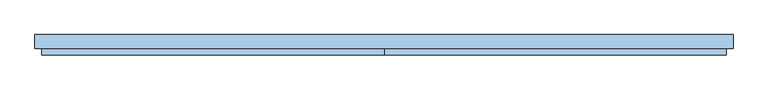
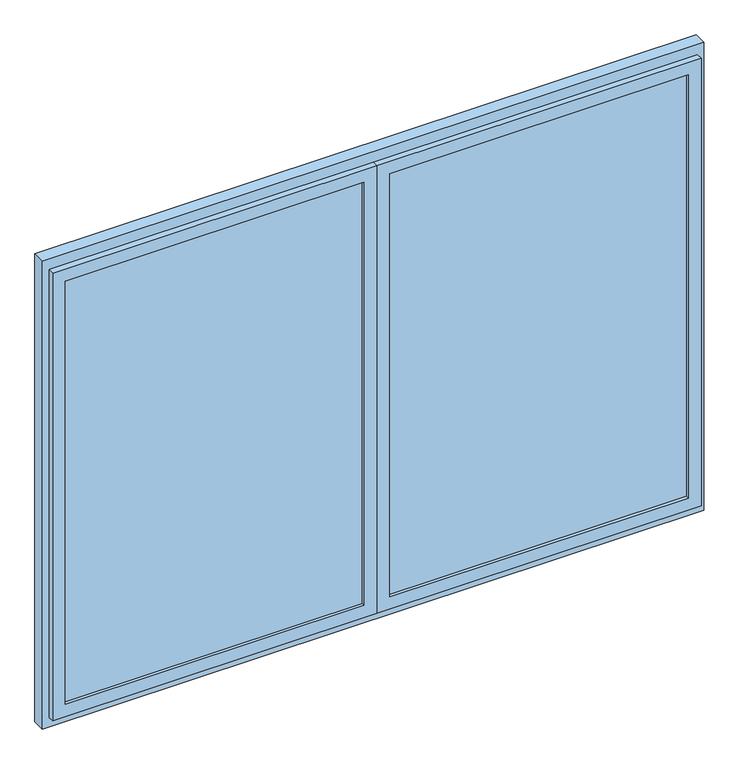
"""IFC4 building model written with IfcOpenShell, lengths in millimetres: window geometry, Fenstertür 2-flg : Fenstertür 2-flg 3.075x2.3."""

import ifcopenshell
import ifcopenshell.guid

model = None  # the IFC model being written
_history = None  # IfcOwnerHistory: only IFC2X3 demands one
_inside = {}  # id of a spatial element -> (the spatial element, [elements in it])
_under = {}  # id of a project, library or spatial element -> (it, [spatial elements below it])
_declared = {}  # id of a project -> (the project, [libraries it declares])
_typed = {}  # id of a type object -> (the type object, [elements of that type])
_made_of = {}  # id of a material, layer set ... -> (it, [elements and type objects made of it])


def new_model(schema):
    """Start an empty IFC model of exactly this schema.

    Asked for "IFC4X3", IfcOpenShell would pick the latest addendum, in which some entities
    have other attributes; the version numbers below select the first issue.
    IFC2X3 requires an IfcOwnerHistory on every rooted entity: one is made here for all.
    """
    global model, _history
    if schema == "IFC4X3":
        model = ifcopenshell.file(schema_version=(4, 3, 0, 0))
    else:
        model = ifcopenshell.file(schema=schema)
    _inside.clear()
    _under.clear()
    _declared.clear()
    _typed.clear()
    _made_of.clear()
    _history = None
    if model.schema == "IFC2X3":
        org = make("IfcOrganization", Name="unknown")
        user = make(
            "IfcPersonAndOrganization",
            ThePerson=make("IfcPerson", FamilyName="unknown"),
            TheOrganization=org,
        )
        app = make(
            "IfcApplication",
            ApplicationDeveloper=org,
            Version="unknown",
            ApplicationFullName="unknown",
            ApplicationIdentifier="unknown",
        )
        _history = make(
            "IfcOwnerHistory",
            OwningUser=user,
            OwningApplication=app,
            ChangeAction="ADDED",
            CreationDate=0,
        )
    return model


def make(cls, **values):
    """One entity of the class cls with the attributes given. An attribute that is None is left unset."""
    return model.create_entity(
        cls, **{name: value for name, value in values.items() if value is not None}
    )


def rooted(cls, **values):
    """An entity with a GlobalId (a new one), such as an element, a storey or a relation."""
    return make(cls, GlobalId=ifcopenshell.guid.new(), OwnerHistory=_history, **values)


def si_unit(unit_type, name, prefix=None):
    """IfcSIUnit, for example si_unit("LENGTHUNIT", "METRE", prefix="MILLI")."""
    return make("IfcSIUnit", UnitType=unit_type, Prefix=prefix, Name=name)


def assignment(units):
    """IfcUnitAssignment: the units of a project."""
    return None if units is None else make("IfcUnitAssignment", Units=units)


def point(xyz):
    """IfcCartesianPoint."""
    return None if xyz is None else make("IfcCartesianPoint", Coordinates=xyz)


def direction(xyz):
    """IfcDirection."""
    return None if xyz is None else make("IfcDirection", DirectionRatios=xyz)


def frame(location, z_axis=None, x_axis=None):
    """IfcAxis2Placement3D, a coordinate frame: its origin and axes. An axis left out is left unset."""
    return make(
        "IfcAxis2Placement3D",
        Location=point(location),
        Axis=direction(z_axis),
        RefDirection=direction(x_axis),
    )


def origin():
    """The frame at (0, 0, 0) with its axes left unset."""
    return frame((0.0, 0.0, 0.0))


def place(relative_to, where):
    """IfcLocalPlacement: puts the frame where relative to a parent placement (None: the world)."""
    return make(
        "IfcLocalPlacement", PlacementRelTo=relative_to, RelativePlacement=where
    )


def context(
    kind, dimensions, precision=None, world=None, true_north=None, identifier=None
):
    """IfcGeometricRepresentationContext, for example the 3D "Model" context."""
    return make(
        "IfcGeometricRepresentationContext",
        ContextIdentifier=identifier,
        ContextType=kind,
        CoordinateSpaceDimension=dimensions,
        Precision=precision,
        WorldCoordinateSystem=world,
        TrueNorth=true_north,
    )


def project(units=None, contexts=None):
    """IfcProject with its units and contexts."""
    return rooted(
        "IfcProject",
        Name="project",
        RepresentationContexts=contexts,
        UnitsInContext=assignment(units),
    )


def spatial(cls, under=None, at=None, **own):
    """A site, building, storey or space (cls), placed at a placement, below another one or the project."""
    s = rooted(cls, ObjectPlacement=at, **own)
    if under is not None:
        _under.setdefault(under.id(), (under, []))[1].append(s)
    return s


def polyline(points):
    """IfcPolyline through the points."""
    return make("IfcPolyline", Points=[point(p) for p in points])


def outline(outer, holes=None, kind="AREA"):
    """IfcArbitraryClosedProfileDef: a profile drawn as a closed curve; with holes, ...WithVoids."""
    if holes is None:
        return make("IfcArbitraryClosedProfileDef", ProfileType=kind, OuterCurve=outer)
    return make(
        "IfcArbitraryProfileDefWithVoids",
        ProfileType=kind,
        OuterCurve=outer,
        InnerCurves=holes,
    )


def extrude(swept, where, along, depth):
    """IfcExtrudedAreaSolid: the profile swept, set in the frame where, extruded along a direction by depth."""
    return make(
        "IfcExtrudedAreaSolid",
        SweptArea=swept,
        Position=where,
        ExtrudedDirection=direction(along),
        Depth=depth,
    )


def faces_of(points, faces, orient=None, outer=None):
    """IfcFace entities. A face is a list of loops; a loop is a list of indices into points, from 0.

    orient and outer hold one flag for each loop. By default every Orientation is true, the
    first loop of a face is its IfcFaceOuterBound and the others are IfcFaceBound.
    """
    made = []
    for i, loops in enumerate(faces):
        bounds = []
        for j, loop in enumerate(loops):
            is_outer = j == 0 if outer is None else outer[i][j]
            bounds.append(
                make(
                    "IfcFaceOuterBound" if is_outer else "IfcFaceBound",
                    Bound=make("IfcPolyLoop", Polygon=[points[k] for k in loop]),
                    Orientation=True if orient is None else orient[i][j],
                )
            )
        made.append(make("IfcFace", Bounds=bounds))
    return made


def faceted_brep(points, faces, orient=None, outer=None, voids=None):
    """IfcFacetedBrep: a solid bounded by flat faces; with voids (closed shells), ...WithVoids."""
    shared = [point(p) for p in points]
    hull = make("IfcClosedShell", CfsFaces=faces_of(shared, faces, orient, outer))
    if voids is None:
        return make("IfcFacetedBrep", Outer=hull)
    return make(
        "IfcFacetedBrepWithVoids",
        Outer=hull,
        Voids=[
            make(cls, CfsFaces=faces_of(shared, fs, o, b)) for cls, fs, o, b in voids
        ],
    )


def shape(context_of_items, identifier, shape_type, items):
    """IfcShapeRepresentation: the items that make up one representation, for example the "Body"."""
    return make(
        "IfcShapeRepresentation",
        ContextOfItems=context_of_items,
        RepresentationIdentifier=identifier,
        RepresentationType=shape_type,
        Items=items,
    )


def source(mapping_origin, context_of_items, identifier, shape_type, items):
    """IfcRepresentationMap: a shape defined once, which mapped items show again and again."""
    return make(
        "IfcRepresentationMap",
        MappingOrigin=mapping_origin,
        MappedRepresentation=shape(context_of_items, identifier, shape_type, items),
    )


def transform(
    local_origin,
    x_axis=None,
    y_axis=None,
    z_axis=None,
    scale=None,
    scale2=None,
    scale3=None,
    uniform=True,
):
    """IfcCartesianTransformationOperator3D, or its non-uniform kind. x_axis, y_axis, z_axis: its Axis1, 2, 3."""
    if uniform:
        return make(
            "IfcCartesianTransformationOperator3D",
            Axis1=direction(x_axis),
            Axis2=direction(y_axis),
            LocalOrigin=point(local_origin),
            Scale=scale,
            Axis3=direction(z_axis),
        )
    return make(
        "IfcCartesianTransformationOperator3DnonUniform",
        Axis1=direction(x_axis),
        Axis2=direction(y_axis),
        LocalOrigin=point(local_origin),
        Scale=scale,
        Axis3=direction(z_axis),
        Scale2=scale2,
        Scale3=scale3,
    )


def mapped(mapping_source, mapping_target):
    """IfcMappedItem: shows the shape of a source again, moved by a transform."""
    return make(
        "IfcMappedItem", MappingSource=mapping_source, MappingTarget=mapping_target
    )


def made_of(thing, what):
    """Note that an element or type object is made of a material, layer set ...; save() writes the relation."""
    if what is not None:
        _made_of.setdefault(what.id(), (what, []))[1].append(thing)
    return thing


def element(
    cls,
    number,
    at=None,
    inside=None,
    cuts=None,
    type_object=None,
    material=None,
    context=None,
    identifier="Body",
    shape_type=None,
    held_by="IfcProductDefinitionShape",
    body=None,
    shapes=None,
    **own,
):
    """One element of the class cls, such as IfcWall. Its Tag is "e" and its number.

    at: its placement. inside: the storey or other place that contains it. cuts: it is an
    opening in that element (IfcRelVoidsElement). A single representation is given by context,
    identifier, shape_type and body (its items); several are given by shapes. held_by: the class
    of the entity that holds the representations. save() writes the other relations.
    """
    e = rooted(cls, Tag="e%d" % number, ObjectPlacement=at, **own)
    if body is not None:
        shapes = [shape(context, identifier, shape_type, body)]
    if shapes is not None:
        e.Representation = make(held_by, Representations=shapes)
    if inside is not None:
        _inside.setdefault(inside.id(), (inside, []))[1].append(e)
    if cuts is not None:
        rooted(
            "IfcRelVoidsElement", RelatingBuildingElement=cuts, RelatedOpeningElement=e
        )
    if type_object is not None:
        _typed.setdefault(type_object.id(), (type_object, []))[1].append(e)
    return made_of(e, material)


def aggregate(whole, parts):
    """IfcRelAggregates: a whole, such as a stair, and the parts it consists of."""
    return rooted("IfcRelAggregates", RelatingObject=whole, RelatedObjects=parts)


def save(model, path):
    """Write the relations noted so far, then the file.

    IfcRelAggregates (storeys below a building ...), IfcRelContainedInSpatialStructure (elements
    in a storey), IfcRelDefinesByType, IfcRelAssociatesMaterial and IfcRelDeclares: one each for
    every whole, place, type object, material and project.
    """
    for whole, parts in _under.values():
        aggregate(whole, parts)
    for where, things in _inside.values():
        rooted(
            "IfcRelContainedInSpatialStructure",
            RelatedElements=things,
            RelatingStructure=where,
        )
    for kind, things in _typed.values():
        rooted("IfcRelDefinesByType", RelatedObjects=things, RelatingType=kind)
    for what, things in _made_of.values():
        rooted("IfcRelAssociatesMaterial", RelatedObjects=things, RelatingMaterial=what)
    for by, libraries in _declared.values():
        rooted("IfcRelDeclares", RelatingContext=by, RelatedDefinitions=libraries)
    model.write(path)


def window_93c93cde(model_context):
    return source(origin(), model_context, "Body", "SolidModel", [
        extrude(outline(polyline([(30.0, -55.0), (-30.0, -55.0), (-30.0, 5.0), (30.0, 5.0), (30.0, -55.0)])), frame((0.0, 0.0, 80.0), z_axis=(0.0, 0.0, 1.0), x_axis=(1.0, 0.0, 0.0)), (0.0, 0.0, 1.0), 2140.0),
        extrude(outline(polyline([(2300.0, -1537.5), (0.0, -1537.5), (0.0, 1537.5), (2300.0, 1537.5), (2300.0, -1537.5)]), holes=[polyline([(2220.0, -1477.5), (2220.0, 1477.5), (80.0, 1477.5), (80.0, -1477.5), (2220.0, -1477.5)])]), frame((0.0, -55.0, 0.0), z_axis=(0.0, 1.0, 0.0), x_axis=(0.0, 0.0, 1.0)), (0.0, 0.0, 1.0), 60.0),
        faceted_brep([(-1477.5, -55.0, 80.0), (-1477.5, -25.0, 80.0), (-30.0, -25.0, 80.0), (-30.0, -55.0, 80.0), (-30.0, -25.0, 2220.0), (-30.0, -55.0, 2220.0), (-1477.5, -25.0, 2220.0), (-60.0, -25.0, 2190.0), (-1447.5, -25.0, 2190.0), (-1447.5, -25.0, 110.0), (-60.0, -25.0, 110.0), (0.0, -55.0, 50.0), (-1507.5, -55.0, 50.0), (-1507.5, -55.0, 2250.0), (0.0, -55.0, 2250.0), (-1477.5, -55.0, 2220.0), (-1507.5, -85.0, 50.0), (0.0, -85.0, 50.0), (0.0, -85.0, 2250.0), (-1507.5, -85.0, 2250.0), (-60.0, -85.0, 110.0), (-1447.5, -85.0, 110.0), (-1447.5, -85.0, 2190.0), (-60.0, -85.0, 2190.0)], [[[0, 1, 2, 3]], [[3, 2, 4, 5]], [[2, 1, 6, 4], [7, 8, 9, 10]], [[11, 12, 13, 14], [5, 15, 0, 3]], [[16, 12, 11, 17]], [[17, 11, 14, 18]], [[18, 19, 16, 17], [20, 21, 22, 23]], [[9, 21, 20, 10]], [[10, 20, 23, 7]], [[15, 6, 1, 0]], [[19, 13, 12, 16]], [[8, 22, 21, 9]], [[5, 4, 6, 15]], [[18, 14, 13, 19]], [[7, 23, 22, 8]]]),
        faceted_brep([(30.0, -55.0, 80.0), (30.0, -25.0, 80.0), (1477.5, -25.0, 80.0), (1477.5, -55.0, 80.0), (1477.5, -25.0, 2220.0), (1477.5, -55.0, 2220.0), (30.0, -25.0, 2220.0), (1447.5, -25.0, 2190.0), (60.0, -25.0, 2190.0), (60.0, -25.0, 110.0), (1447.5, -25.0, 110.0), (1507.5, -55.0, 50.0), (0.0, -55.0, 50.0), (0.0, -55.0, 2250.0), (1507.5, -55.0, 2250.0), (30.0, -55.0, 2220.0), (0.0, -85.0, 50.0), (1507.5, -85.0, 50.0), (1507.5, -85.0, 2250.0), (0.0, -85.0, 2250.0), (1447.5, -85.0, 110.0), (60.0, -85.0, 110.0), (60.0, -85.0, 2190.0), (1447.5, -85.0, 2190.0)], [[[0, 1, 2, 3]], [[3, 2, 4, 5]], [[2, 1, 6, 4], [7, 8, 9, 10]], [[11, 12, 13, 14], [5, 15, 0, 3]], [[16, 12, 11, 17]], [[17, 11, 14, 18]], [[18, 19, 16, 17], [20, 21, 22, 23]], [[9, 21, 20, 10]], [[10, 20, 23, 7]], [[15, 6, 1, 0]], [[19, 13, 12, 16]], [[8, 22, 21, 9]], [[5, 4, 6, 15]], [[18, 14, 13, 19]], [[7, 23, 22, 8]]]),
        extrude(outline(polyline([(60.0, -40.0), (1447.5, -40.0), (1447.5, -70.0), (60.0, -70.0), (60.0, -40.0)])), frame((0.0, 0.0, 110.0), z_axis=(0.0, 0.0, 1.0), x_axis=(1.0, 0.0, 0.0)), (0.0, 0.0, 1.0), 2080.0),
        extrude(outline(polyline([(-1447.5, -40.0), (-60.0, -40.0), (-60.0, -70.0), (-1447.5, -70.0), (-1447.5, -40.0)])), frame((0.0, 0.0, 110.0), z_axis=(0.0, 0.0, 1.0), x_axis=(1.0, 0.0, 0.0)), (0.0, 0.0, 1.0), 2080.0),
    ])


if __name__ == "__main__":
    model = new_model("IFC4")
    model_context = context("Model", 3, world=origin())
    ifc_project = project(units=[si_unit("LENGTHUNIT", "METRE", prefix="MILLI")], contexts=[model_context])
    site = spatial("IfcSite", under=ifc_project)
    building = spatial("IfcBuilding", under=site)
    placement = place(None, origin())
    window_shape = window_93c93cde(model_context)
    element("IfcWindow", 1, ObjectType="Fenstertür 2-flg : Fenstertür 2-flg 3.075x2.3", at=placement, inside=building, context=model_context, shape_type="MappedRepresentation", body=[
        mapped(window_shape, transform((0.0, 0.0, 0.0), x_axis=(1.0, 0.0, 0.0), y_axis=(0.0, 1.0, 0.0), z_axis=(0.0, 0.0, 1.0))),
    ])
    save(model, "model.ifc")

# Revit data of these elements
# Type "Fenstertür 2-flg : Fenstertür 2-flg 3.075x2.3"
#   Type Mark = "75"
#   Operation = "DoublePanelVertical"
#   Construction Type Id = "GSP4R"
#   Keynote = "16.05.01"
#   Analytic Construction = "1/8 Zoll Pilkington-Verglasung einfach"
#   Thermal Resistance (R) = 0.271106 (m²·K)/W
#   Visual Light Transmittance = 0.9
#   Solar Heat Gain Coefficient = 0.78
#   Rough Width = 3.075 m
#   Rough Height = 2.300 m
#   Heat Transfer Coefficient (U) = 3.6886 W/(m²·K)
#   Rahmentiefe = 0.060 m
#   Rahmenhöhe unten = 0.080 m
#   Höhe oberer  Rahmen = 0.080 m
#   Rahmenbreite = 0.060 m
#   Height = 2.300 m
#   Tiefe Flügel = 0.060 m
#   Flügelbreite = 0.060 m
#   Einbautiefe (von außen) [instance default] = 0.140 m
#   Width = 3.075 m
#   Sichtbarkeit Sturzlinien [instance default] = yes
#   Öffnungsrichtung oben [instance default] = yes
#   Öffnungsrichtung in Draufsicht anzeigen [instance default] = yes
#   Drehflügel 1 [instance default] = yes
#   Bild [instance default] = none
#   Glas [instance default] = none
#   Fensterflügel [instance default] = none
#   Äußere Fensterbank [instance default] = none
#   Innere Fensterbank [instance default] = none
#   Wall Closure = (empty or 0)
# Element 1 (IfcWindow, "Fenstertür 2-flg : Fenstertür 2-flg 3.075x2.3")
#   Einbautiefe (von außen) = 0.220 m
#   Materials on its faces: "Kunststoff - Weiß", "Glas"
# Materials
#   "Kunststoff - Weiß": class "Kunststoff", colour RGB 249 249 249, transparency 0, Cost = 0
#   "Glas": class "Glas", colour RGB 0 0 255, transparency 0.75, Comments = "Render-Darstellung nicht aktualisiert ", Cost = 0
